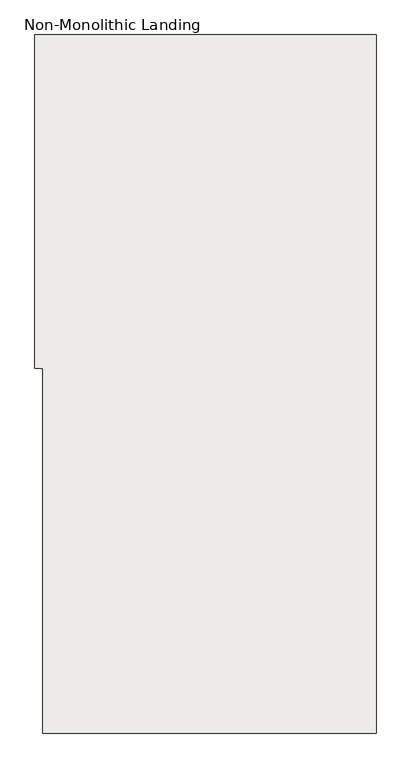
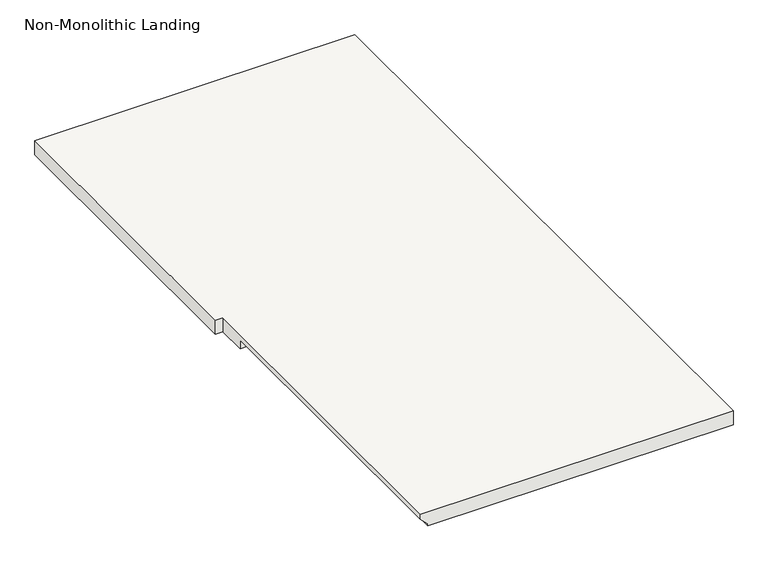
"""IFC4 building model written with IfcOpenShell, lengths in millimetres: slab geometry, Non-Monolithic Landing."""

from ifc_helpers import new_model, si_unit, origin, place, context, project, spatial, faceted_brep, source, transform, mapped, element, save


def non_monolithic_landing_34ebcfd1(model_context):
    return source(origin(), model_context, "Body", "Brep", [
        faceted_brep([(665981.788677, -551651.2413841, 4626.4040541), (665956.388677, -551651.2413841, 4651.8040541), (665956.388677, -550584.4413841, 4651.8040541), (665981.788677, -550584.4413841, 4626.4040541), (667023.188677, -551651.2413841, 4670.8540541), (667023.188677, -549416.0413841, 4670.8540541), (665956.388677, -549416.0413841, 4670.8540541), (665930.988677, -549416.0413841, 4670.8540541), (665930.988677, -550482.8413841, 4670.8540541), (665956.388677, -550482.8413841, 4670.8540541), (665956.388677, -551651.2413841, 4670.8540541), (665981.788677, -550584.4413841, 4620.0540541), (665956.388677, -550584.4413841, 4620.0540541), (665956.388677, -550482.8413841, 4620.0540541), (665930.988677, -550482.8413841, 4620.0540541), (665930.988677, -549416.0413841, 4620.0540541), (665956.388677, -549416.0413841, 4620.0540541), (667023.188677, -549416.0413841, 4620.0540541), (667023.188677, -551651.2413841, 4620.0540541), (665981.788677, -551651.2413841, 4620.0540541)], [[[0, 1, 2, 3]], [[4, 5, 6, 7, 8, 9, 10]], [[11, 12, 13, 14, 15, 16, 17, 18, 19]], [[12, 11, 3, 2]], [[11, 19, 0, 3]], [[4, 10, 1, 0, 19, 18]], [[5, 4, 18, 17]], [[6, 5, 17, 16]], [[7, 6, 16, 15]], [[8, 7, 15, 14]], [[9, 8, 14, 13]], [[10, 9, 13, 12, 2, 1]]]),
    ])


if __name__ == "__main__":
    model = new_model("IFC4")
    model_context = context("Model", 3, world=origin())
    ifc_project = project(units=[si_unit("LENGTHUNIT", "METRE", prefix="MILLI")], contexts=[model_context])
    site = spatial("IfcSite", under=ifc_project)
    building = spatial("IfcBuilding", under=site)
    placement = place(None, origin())
    non_monolithic_landing_shape = non_monolithic_landing_34ebcfd1(model_context)
    element("IfcSlab", 1, ObjectType="Non-Monolithic Landing", at=placement, inside=building, context=model_context, shape_type="MappedRepresentation", body=[
        mapped(non_monolithic_landing_shape, transform((0.0, 0.0, 0.0), x_axis=(1.0, 0.0, 0.0), y_axis=(0.0, 1.0, 0.0), z_axis=(0.0, 0.0, 1.0))),
    ])
    save(model, "model.ifc")
